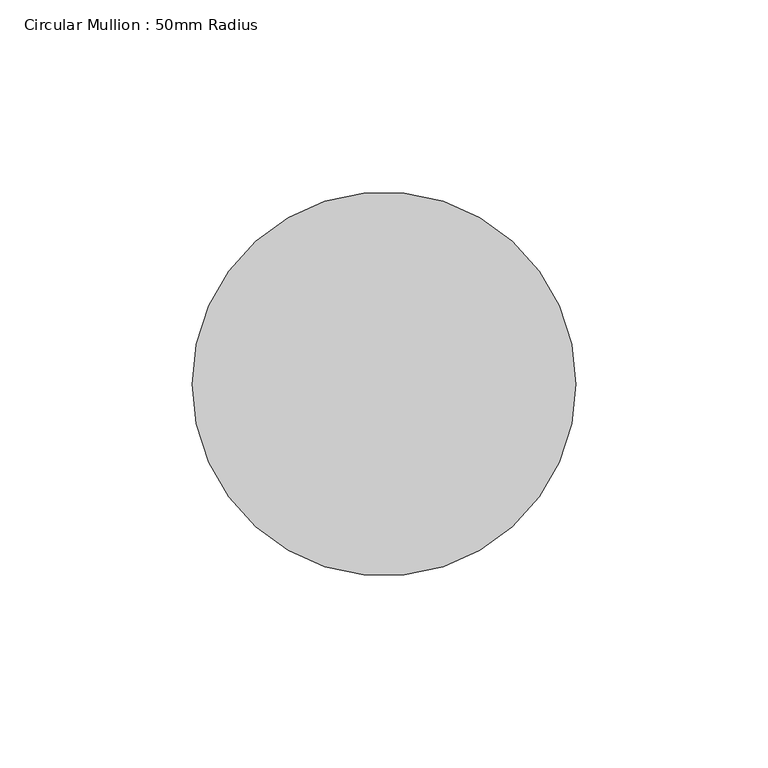
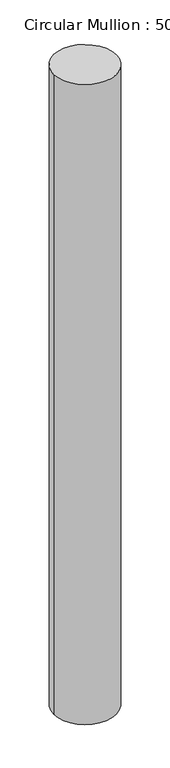
"""IFC4 building model written with IfcOpenShell, lengths in millimetres: member geometry, Circular Mullion : 50mm Radius."""

from ifc_helpers import new_model, si_unit, frame, origin, place, context, project, spatial, ellipse_curve, source, transform, mapped, element, save
from ifc_brep_helpers import plane_surface, cylinder_surface, advanced_brep


def circular_mullion_50mm_radius_69de481d(model_context):
    return source(origin(), model_context, "Body", "AdvancedBrep", [
        advanced_brep(
        [(-100.0, 0.0, 1.1774236), (0.0, 0.0, 0.0), (0.0, 0.0, -1085.2319928), (-100.0, 0.0, -1086.4462241)],
        [
            (0, 1, ellipse_curve(frame((-50.0, 0.0, 0.5887118), z_axis=(-0.01177208018429299, -0.015085939052492408, -0.9998168995226272), x_axis=(-0.6150831494596131, -0.7882300120027672, 0.01913550179537054)), 50.0091567, 50.0)),
            (1, 2),
            (2, 3, ellipse_curve(frame((-50.0, 0.0, -1085.8391084), z_axis=(-0.012139948487221193, -0.015557362854442007, 0.9998052760971723), x_axis=(0.6150759987771495, 0.7882208483921463, 0.01973347126729143)), 50.0097381, 50.0)),
            (3, 0),
            (1, 0, ellipse_curve(frame((-50.0, 0.0, 0.5887118), z_axis=(-0.01177208018429299, -0.015085939052492408, -0.9998168995226272), x_axis=(-0.6150831494596131, -0.7882300120027672, 0.01913550179537054)), 50.0091567, 50.0)),
            (3, 2, ellipse_curve(frame((-50.0, 0.0, -1085.8391084), z_axis=(-0.012139948487221193, -0.015557362854442007, 0.9998052760971723), x_axis=(0.6150759987771495, 0.7882208483921463, 0.01973347126729143)), 50.0097381, 50.0)),
        ],
        [
            cylinder_surface(frame((-50.0, 0.0, 0.0), z_axis=(0.0, 0.0, 1.0), x_axis=(1.0, 0.0, 0.0)), 50.0),
            plane_surface(frame((-240.2965061, 187.5116774, 0.0), z_axis=(0.01177208018429299, 0.015085939052492408, 0.9998168995226272), x_axis=(0.615083149459613, 0.7882300120027673, -0.01913550179537864))),
            plane_surface(frame((-240.2965061, 187.5116774, -1085.2319928), z_axis=(0.012139948487221193, 0.015557362854442007, -0.9998052760971723), x_axis=(0.6150759987771495, 0.7882208483921463, 0.019733471267294966))),
        ],
        [
            (0, [[1, 2, 3, 4]]),
            (0, [[5, -4, 6, -2]]),
            (1, [[-1, -5]]),
            (2, [[-6, -3]]),
        ],
    ),
    ])


if __name__ == "__main__":
    model = new_model("IFC4")
    model_context = context("Model", 3, world=origin())
    ifc_project = project(units=[si_unit("LENGTHUNIT", "METRE", prefix="MILLI")], contexts=[model_context])
    site = spatial("IfcSite", under=ifc_project)
    building = spatial("IfcBuilding", under=site)
    placement = place(None, origin())
    circular_mullion_50mm_radius_shape = circular_mullion_50mm_radius_69de481d(model_context)
    element("IfcMember", 1, ObjectType="Circular Mullion : 50mm Radius", at=placement, inside=building, context=model_context, shape_type="MappedRepresentation", body=[
        mapped(circular_mullion_50mm_radius_shape, transform((0.0, 0.0, 0.0), x_axis=(1.0, 0.0, 0.0), y_axis=(0.0, 1.0, 0.0), z_axis=(0.0, 0.0, 1.0))),
    ])
    save(model, "model.ifc")

# Revit data of these elements
# Type "Circular Mullion : 50mm Radius"
#   built-in parameter 1007350 = 0.164042 (stored number, unit not read)
# Element 1 (IfcMember, "Circular Mullion : 50mm Radius")
#   Materials on its faces: "Aluminium"
# Materials
#   "Aluminium": class "Metal", colour RGB 247 247 247, transparency 0, Description = "Aluminium 6061", Cost = 0
